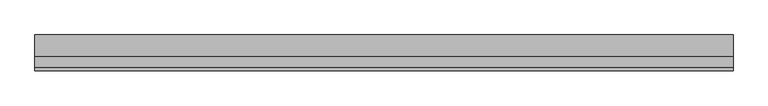
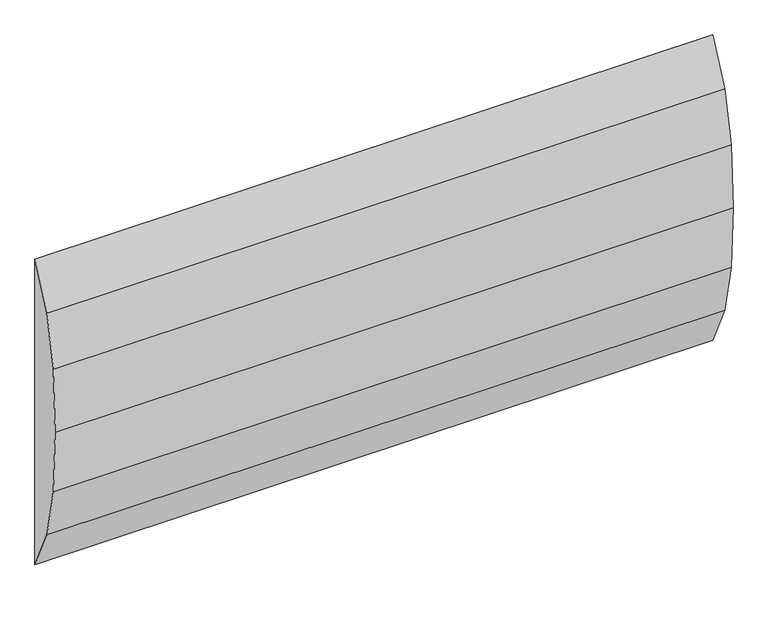
"""IFC4 building model written with IfcOpenShell, lengths in millimetres: proxy geometry, Generic Models 7:Generic Models 1:337419:Generic Models 1:337419 : Generic Models 7:Generic Models 1:337419:14 : Generic Models 7:Generic Models 1:337419:Generic Models 1:337419 : Generic Models 7:Generic Models 1:337419:301336."""

from ifc_helpers import new_model, si_unit, frame, origin, place, context, project, spatial, polyline, outline, extrude, source, transform, mapped, element, save


def generic_models_b760832c(model_context):
    return source(origin(), model_context, "Body", "SweptSolid", [
        extrude(outline(polyline([(-536693.7909841, 4050.485356), (-536775.398255, 4427.1461193), (-536796.2774202, 4891.3851563), (-536775.398255, 5355.6241932), (-536693.7909841, 5732.2849565), (-536544.5913841, 6052.2445313), (-536544.5913841, 3730.5257813), (-536693.7909841, 4050.485356)])), frame((597433.7867239, 0.0, 0.0), z_axis=(1.0, 0.0, 0.0), x_axis=(0.0, 1.0, 0.0)), (0.0, 0.0, 1.0), 4876.8),
    ])


if __name__ == "__main__":
    model = new_model("IFC4")
    model_context = context("Model", 3, world=origin())
    ifc_project = project(units=[si_unit("LENGTHUNIT", "METRE", prefix="MILLI")], contexts=[model_context])
    site = spatial("IfcSite", under=ifc_project)
    building = spatial("IfcBuilding", under=site)
    placement = place(None, origin())
    generic_models_shape = generic_models_b760832c(model_context)
    element("IfcBuildingElementProxy", 1, Name="Generic Models 7:Generic Models 1:337419:Generic Models 1:337419 : Generic Models 7:Generic Models 1:337419:14 : Generic Models 7:Generic Models 1:337419:Generic Models 1:337419 : Generic Models 7:Generic Models 1:337419:301336", ObjectType="Generic Models 7:Generic Models 1:337419:Generic Models 1:337419 : Generic Models 7:Generic Models 1:337419:14 : Generic Models 7:Generic Models 1:337419:Generic Models 1:337419 : Generic Models 7:Generic Models 1:337419:301336", at=placement, inside=building, context=model_context, shape_type="MappedRepresentation", body=[
        mapped(generic_models_shape, transform((0.0, 0.0, 0.0), x_axis=(1.0, 0.0, 0.0), y_axis=(0.0, 1.0, 0.0), z_axis=(0.0, 0.0, 1.0))),
    ])
    save(model, "model.ifc")

# Revit data of these elements
# Type "Generic Models 7:Generic Models 1:337419:Generic Models 1:337419 : Generic Models 7:Generic Models 1:337419:14 : Generic Models 7:Generic Models 1:337419:Generic Models 1:337419 : Generic Models 7:Generic Models 1:337419:301336"
#   NameOverride = "Generic Models 7:Generic Models 1:337419:Generic Models 1:337419 : Generic Models 7:Generic Models 1:337419:301336"
#   ObjectTypeOverride = "Generic Models 1:337419 : Generic Models 7:Generic Models 1:337419"
#   Reference = "Generic Models 1"
#   Tag = "301336"
# Element 1 (IfcBuildingElementProxy, "Generic Models 7:Generic Models 1:337419:Generic Models 1:337419 : Generic Models 7:Generic Models 1:337419:14 : Generic Models 7:Generic Models 1:337419:Generic Models 1:337419 : Generic Models 7:Generic Models 1:337419:301336")
#   Materials on its faces: "SIMPLE SAVER INSULATION WITH LINER - COLOR: WHITE"
# Materials
#   "SIMPLE SAVER INSULATION WITH LINER - COLOR: WHITE": class "Unassigned", colour RGB 219 193 225, transparency 0, Cost = 0
